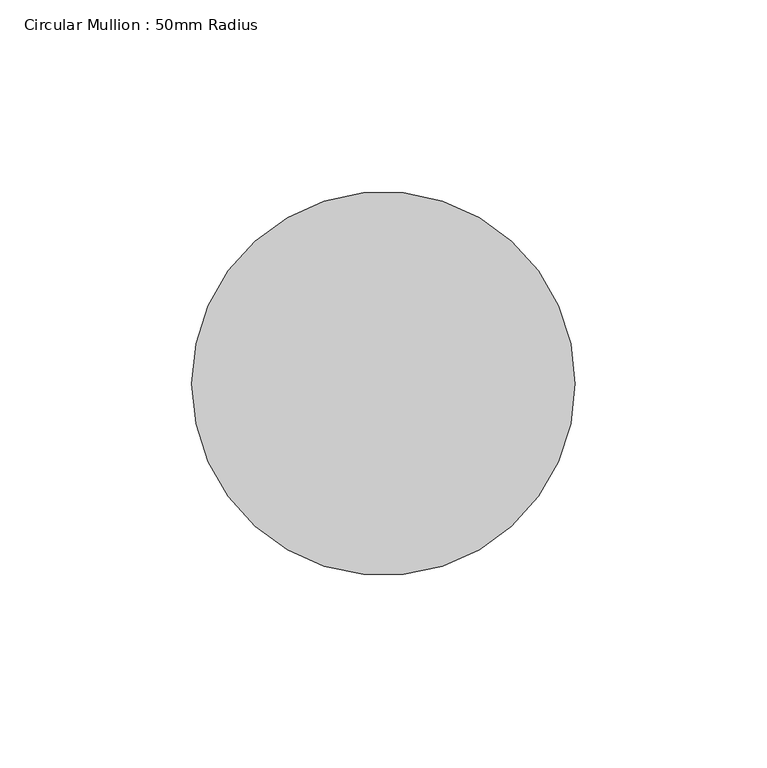
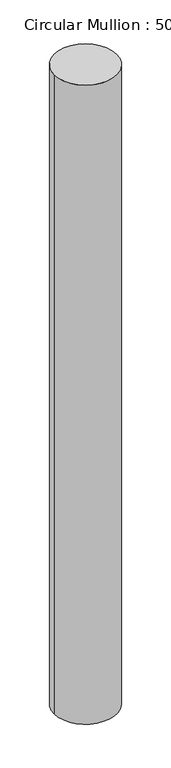
"""IFC4 building model written with IfcOpenShell, lengths in millimetres: member geometry, Circular Mullion : 50mm Radius."""

from ifc_helpers import new_model, si_unit, point, frame, origin, origin_2d, place, context, project, spatial, circle_curve, trimmed, segment, composite_curve, outline, extrude, source, transform, mapped, element, save


def circular_mullion_50mm_radius_8295ec6c(model_context):
    return source(origin(), model_context, "Body", "SweptSolid", [
        extrude(outline(composite_curve([segment(trimmed(circle_curve(origin_2d(), 50.0), [point((50.0, 0.0))], [point((-50.0, 0.0))], False, "CARTESIAN"), True, "CONTINUOUS"), segment(trimmed(circle_curve(origin_2d(), 50.0), [point((-50.0, 0.0))], [point((50.0, 0.0))], False, "CARTESIAN"), True, "CONTINUOUS")], self_intersect=False)), frame((0.0, 0.0, -1077.8364553), z_axis=(0.0, 0.0, 1.0), x_axis=(1.0, 0.0, 0.0)), (0.0, 0.0, 1.0), 1077.8364553),
    ])


if __name__ == "__main__":
    model = new_model("IFC4")
    model_context = context("Model", 3, world=origin())
    ifc_project = project(units=[si_unit("LENGTHUNIT", "METRE", prefix="MILLI")], contexts=[model_context])
    site = spatial("IfcSite", under=ifc_project)
    building = spatial("IfcBuilding", under=site)
    placement = place(None, origin())
    circular_mullion_50mm_radius_shape = circular_mullion_50mm_radius_8295ec6c(model_context)
    element("IfcMember", 1, ObjectType="Circular Mullion : 50mm Radius", at=placement, inside=building, context=model_context, shape_type="MappedRepresentation", body=[
        mapped(circular_mullion_50mm_radius_shape, transform((0.0, 0.0, 0.0), x_axis=(1.0, 0.0, 0.0), y_axis=(0.0, 1.0, 0.0), z_axis=(0.0, 0.0, 1.0))),
    ])
    save(model, "model.ifc")

# Revit data of these elements
# Type "Circular Mullion : 50mm Radius"
#   built-in parameter 1007350 = 0.164042 (stored number, unit not read)
# Element 1 (IfcMember, "Circular Mullion : 50mm Radius")
#   Materials on its faces: "Aluminium"
# Materials
#   "Aluminium": class "Metal", colour RGB 247 247 247, transparency 0, Description = "Aluminium 6061", Cost = 0
